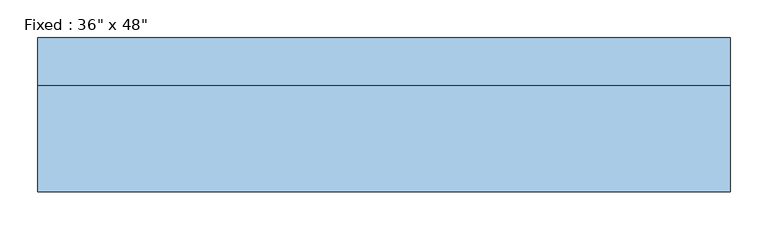
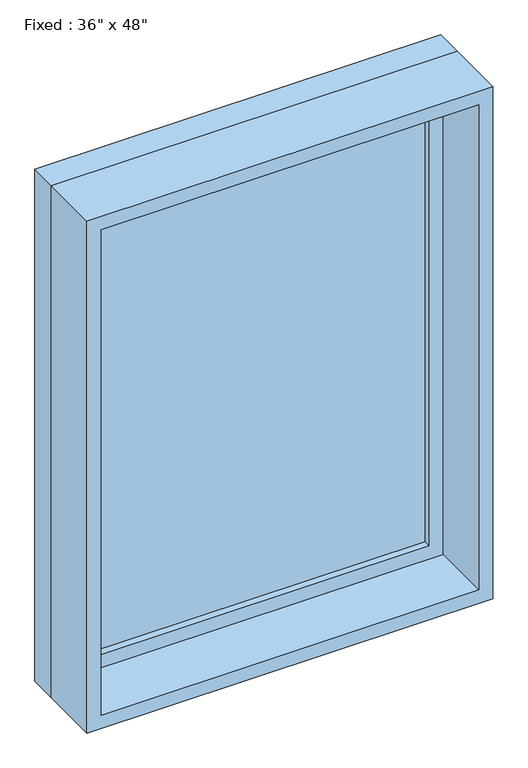
"""IFC4 building model written with IfcOpenShell, lengths in millimetres: window geometry."""

from ifc_helpers import new_model, si_unit, frame, origin, place, context, project, spatial, polyline, outline, extrude, source, transform, mapped, element, save


def window_e2841890(model_context):
    return source(origin(), model_context, "Body", "SweptSolid", [
        extrude(outline(polyline([(355.6, 53.975), (-431.8, 53.975), (-431.8, 66.675), (355.6, 66.675), (355.6, 53.975)])), frame((0.0, 0.0, 977.9), z_axis=(0.0, 0.0, 1.0), x_axis=(1.0, 0.0, 0.0)), (0.0, 0.0, 1.0), 1092.2),
        extrude(outline(polyline([(2114.55, -476.25), (933.45, -476.25), (933.45, 400.05), (2114.55, 400.05), (2114.55, -476.25)]), holes=[polyline([(2070.1, -431.8), (2070.1, 355.6), (977.9, 355.6), (977.9, -431.8), (2070.1, -431.8)])]), frame((0.0, 38.1, 0.0), z_axis=(0.0, 1.0, 0.0), x_axis=(0.0, 0.0, 1.0)), (0.0, 0.0, 1.0), 44.45),
        extrude(outline(polyline([(2133.6, -495.3), (914.4, -495.3), (914.4, 419.1), (2133.6, 419.1), (2133.6, -495.3)]), holes=[polyline([(2101.85, -463.55), (2101.85, 387.35), (946.15, 387.35), (946.15, -463.55), (2101.85, -463.55)])]), frame((0.0, -101.6, 0.0), z_axis=(0.0, 1.0, 0.0), x_axis=(0.0, 0.0, 1.0)), (0.0, 0.0, 1.0), 139.7),
        extrude(outline(polyline([(2133.6, 419.1), (2133.6, -495.3), (914.4, -495.3), (914.4, 419.1), (2133.6, 419.1)]), holes=[polyline([(2114.55, 400.05), (933.45, 400.05), (933.45, -476.25), (2114.55, -476.25), (2114.55, 400.05)])]), frame((0.0, 38.1, 0.0), z_axis=(0.0, 1.0, 0.0), x_axis=(0.0, 0.0, 1.0)), (0.0, 0.0, 1.0), 63.5),
    ])


if __name__ == "__main__":
    model = new_model("IFC4")
    model_context = context("Model", 3, world=origin())
    ifc_project = project(units=[si_unit("LENGTHUNIT", "METRE", prefix="MILLI")], contexts=[model_context])
    site = spatial("IfcSite", under=ifc_project)
    building = spatial("IfcBuilding", under=site)
    placement = place(None, origin())
    window_shape = window_e2841890(model_context)
    element("IfcWindow", 1, ObjectType="Fixed : 36\" x 48\"", at=placement, inside=building, context=model_context, shape_type="MappedRepresentation", body=[
        mapped(window_shape, transform((0.0, 0.0, 0.0), x_axis=(1.0, 0.0, 0.0), y_axis=(0.0, 1.0, 0.0), z_axis=(0.0, 0.0, 1.0))),
    ])
    save(model, "model.ifc")

# Revit data of these elements
# Type "Fixed : 36\" x 48\""
#   Type Mark = "1"
#   Construction Type Id = "GSP4R"
#   Assembly Code = "B2020100"
#   Analytic Construction = "1/8 in Pilkington single glazing"
#   Visual Light Transmittance = 0.9
#   Solar Heat Gain Coefficient = 0.78
#   Heat Transfer Coefficient (U) = 0.6496 BTU/(h·ft²·°F)
#   Height = 4' - 0"
#   Default Sill Height = 3' - 0"
#   Width = 3' - 0"
#   Window Inset = 0' - 0 3/4"
#   Define Thermal Properties by = 1
#   Define Thermal Properties by = 1
#   Glass Pane Material = Glass
#   Sash Material = Sash
#   Wall Closure = (empty or 0)
# Element 1 (IfcWindow, "Fixed : 36\" x 48\"")
#   Materials on its faces: "Sash", "Glass"
# Materials
#   "Glass": class "Glass", colour RGB 0 128 192, transparency 0.75, Description = "Soda Lime Glass", Cost = 0
#   "Sash": class "Wood", colour RGB 224 178 126, transparency 0, Cost = 0
